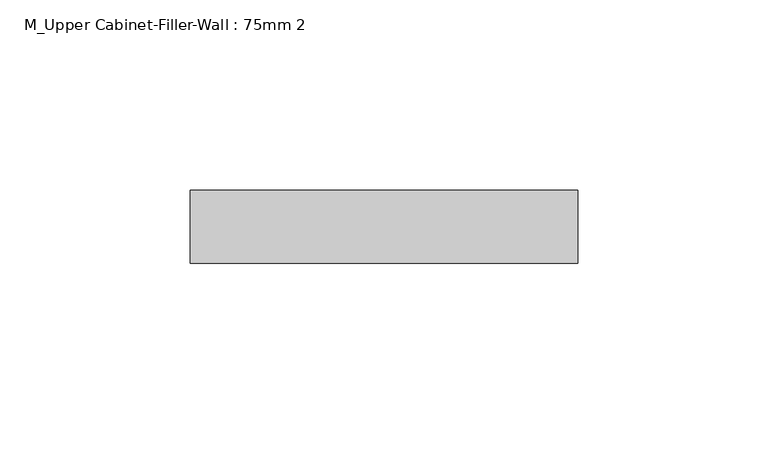
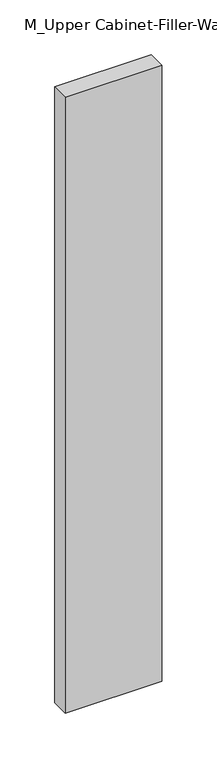
"""IFC4 building model written with IfcOpenShell, lengths in millimetres: furniture geometry, M_Upper Cabinet-Filler-Wall : 75mm 2."""

from ifc_helpers import new_model, si_unit, frame, origin, place, context, project, spatial, polyline, outline, extrude, source, transform, mapped, element, save


def m_upper_cabinet_filler_wall_75mm_2_2fb8ce97(model_context):
    return source(origin(), model_context, "Body", "SweptSolid", [
        extrude(outline(polyline([(-21.0288372, 88.9), (-21.0288372, 107.95), (80.5711628, 107.95), (80.5711628, 88.9), (-21.0288372, 88.9)])), frame((0.0, 0.0, 1314.1523437), z_axis=(0.0, 0.0, 1.0), x_axis=(1.0, 0.0, 0.0)), (0.0, 0.0, 1.0), 685.8),
    ])


if __name__ == "__main__":
    model = new_model("IFC4")
    model_context = context("Model", 3, world=origin())
    ifc_project = project(units=[si_unit("LENGTHUNIT", "METRE", prefix="MILLI")], contexts=[model_context])
    site = spatial("IfcSite", under=ifc_project)
    building = spatial("IfcBuilding", under=site)
    placement = place(None, origin())
    m_upper_cabinet_filler_wall_75mm_2_shape = m_upper_cabinet_filler_wall_75mm_2_2fb8ce97(model_context)
    element("IfcFurniture", 1, ObjectType="M_Upper Cabinet-Filler-Wall : 75mm 2", at=placement, inside=building, context=model_context, shape_type="MappedRepresentation", body=[
        mapped(m_upper_cabinet_filler_wall_75mm_2_shape, transform((0.0, 0.0, 0.0), x_axis=(1.0, 0.0, 0.0), y_axis=(0.0, 1.0, 0.0), z_axis=(0.0, 0.0, 1.0))),
    ])
    save(model, "model.ifc")

# Revit data of these elements
# Type "M_Upper Cabinet-Filler-Wall : 75mm 2"
#   Depth = 0' - 3"
#   Height = 2' - 3"
#   Top Of Cabinet = 6' - 6 189/256"
#   Width = 0' - 4"
#   Cabinet Material = none
#   Default Elevation = 0
# Element 1 (IfcFurniture, "M_Upper Cabinet-Filler-Wall : 75mm 2")
#   Materials on its faces: "Cabinets"
# Materials
#   "Cabinets": class "Miscellaneous", colour RGB 249 249 249, transparency 0
